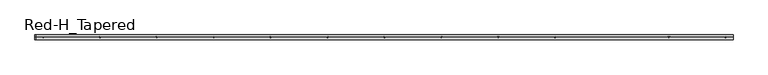
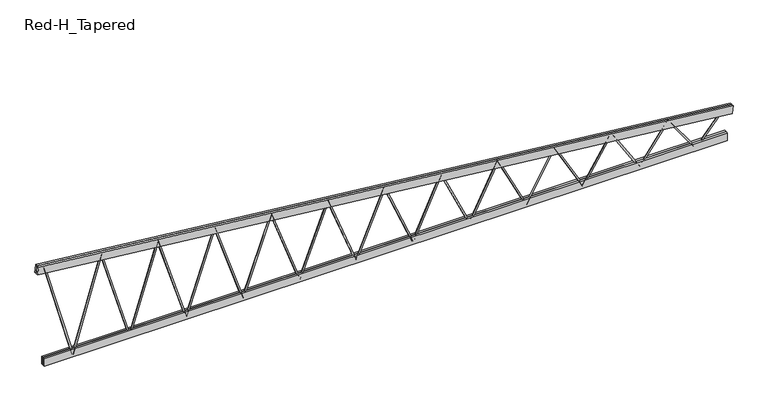
"""IFC4 building model written with IfcOpenShell, lengths in millimetres: beam geometry, Construction_Frames_RedBuilt_Openweb_Red-H_Tapered : Red-H_Tapered."""

from ifc_helpers import new_model, si_unit, point, frame, origin, origin_2d, place, context, project, spatial, polyline, circle_curve, trimmed, segment, composite_curve, outline, extrude, source, transform, mapped, element, save


def red_h_tapered_72d70656(model_context):
    return source(origin(), model_context, "Body", "SweptSolid", [
        extrude(outline(composite_curve([segment(trimmed(circle_curve(origin_2d(), 12.7), [point((0.0, -12.7000001))], [point((0.0, 12.7))], False, "CARTESIAN"), True, "CONTINUOUS"), segment(trimmed(circle_curve(origin_2d(), 12.7), [point((0.0, 12.7))], [point((0.0, -12.7000001))], False, "CARTESIAN"), True, "CONTINUOUS")], self_intersect=False)), frame((-495.696875, 0.0, -367.0101562), z_axis=(-0.36126696231281513, 0.0, 0.9324624292384498), x_axis=(0.0, -1.0, 0.0)), (0.0, 0.0, 1.0), 1372.1068537),
        extrude(outline(composite_curve([segment(trimmed(circle_curve(origin_2d(), 12.7), [point((0.0, 12.7000001))], [point((0.0, -12.7))], False, "CARTESIAN"), True, "CONTINUOUS"), segment(trimmed(circle_curve(origin_2d(), 12.7), [point((0.0, -12.7))], [point((0.0, 12.7000001))], False, "CARTESIAN"), True, "CONTINUOUS")], self_intersect=False)), frame((-1487.090625, 0.0, -367.0101562), z_axis=(0.3612669623128153, 0.0, 0.9324624292384498), x_axis=(0.0, -1.0, 0.0)), (0.0, 0.0, 1.0), 1372.1068537),
        extrude(outline(composite_curve([segment(trimmed(circle_curve(origin_2d(), 12.7), [point((0.0, -12.7000001))], [point((0.0, 12.7))], False, "CARTESIAN"), True, "CONTINUOUS"), segment(trimmed(circle_curve(origin_2d(), 12.7), [point((0.0, 12.7))], [point((0.0, -12.7000001))], False, "CARTESIAN"), True, "CONTINUOUS")], self_intersect=False)), frame((-1487.090625, 0.0, -367.0101562), z_axis=(-0.33832311058632253, 0.0, 0.9410300063458099), x_axis=(0.0, -1.0, 0.0)), (0.0, 0.0, 1.0), 1465.158186),
        extrude(outline(composite_curve([segment(trimmed(circle_curve(origin_2d(), 12.7), [point((0.0, -12.7))], [point((0.0, 12.7000001))], False, "CARTESIAN"), True, "CONTINUOUS"), segment(trimmed(circle_curve(origin_2d(), 12.7), [point((0.0, 12.7000001))], [point((0.0, -12.7))], False, "CARTESIAN"), True, "CONTINUOUS")], self_intersect=False)), frame((-2478.484375, 0.0, -367.0101562), z_axis=(0.3383231105863266, 0.0, 0.9410300063458085), x_axis=(0.0, -1.0, 0.0)), (0.0, 0.0, 1.0), 1465.158186),
        extrude(outline(composite_curve([segment(trimmed(circle_curve(origin_2d(), 12.7), [point((0.0, 12.7))], [point((0.0, -12.7))], False, "CARTESIAN"), True, "CONTINUOUS"), segment(trimmed(circle_curve(origin_2d(), 12.7), [point((0.0, -12.7))], [point((0.0, 12.7))], False, "CARTESIAN"), True, "CONTINUOUS")], self_intersect=False)), frame((-2478.484375, 0.0, -367.0101562), z_axis=(-0.3179616527746543, 0.0, 0.9481035741757387), x_axis=(0.0, -1.0, 0.0)), (0.0, 0.0, 1.0), 1558.9832003),
        extrude(outline(composite_curve([segment(trimmed(circle_curve(origin_2d(), 12.7), [point((0.0, -12.7))], [point((0.0, 12.7))], False, "CARTESIAN"), True, "CONTINUOUS"), segment(trimmed(circle_curve(origin_2d(), 12.7), [point((0.0, 12.7))], [point((0.0, -12.7))], False, "CARTESIAN"), True, "CONTINUOUS")], self_intersect=False)), frame((-3469.878125, 0.0, -367.0101562), z_axis=(0.3179616527746538, 0.0, 0.9481035741757388), x_axis=(0.0, -1.0, 0.0)), (0.0, 0.0, 1.0), 1558.9832003),
        extrude(outline(composite_curve([segment(trimmed(circle_curve(origin_2d(), 12.7), [point((0.0, 12.6999999))], [point((0.0, -12.7))], False, "CARTESIAN"), True, "CONTINUOUS"), segment(trimmed(circle_curve(origin_2d(), 12.7), [point((0.0, -12.7))], [point((0.0, 12.6999999))], False, "CARTESIAN"), True, "CONTINUOUS")], self_intersect=False)), frame((-3469.878125, 0.0, -367.0101562), z_axis=(-0.29979546818875297, 0.0, 0.9540034996023267), x_axis=(0.0, -1.0, 0.0)), (0.0, 0.0, 1.0), 1653.4501939),
        extrude(outline(composite_curve([segment(trimmed(circle_curve(origin_2d(), 12.7), [point((0.0, -12.6999999))], [point((0.0, 12.7))], False, "CARTESIAN"), True, "CONTINUOUS"), segment(trimmed(circle_curve(origin_2d(), 12.7), [point((0.0, 12.7))], [point((0.0, -12.6999999))], False, "CARTESIAN"), True, "CONTINUOUS")], self_intersect=False)), frame((-4461.271875, 0.0, -367.0101562), z_axis=(0.29979546818875863, 0.0, 0.9540034996023249), x_axis=(0.0, -1.0, 0.0)), (0.0, 0.0, 1.0), 1653.4501939),
        extrude(outline(composite_curve([segment(trimmed(circle_curve(origin_2d(), 12.7), [point((0.0, 12.6999999))], [point((0.0, -12.7))], False, "CARTESIAN"), True, "CONTINUOUS"), segment(trimmed(circle_curve(origin_2d(), 12.7), [point((0.0, -12.7))], [point((0.0, 12.6999999))], False, "CARTESIAN"), True, "CONTINUOUS")], self_intersect=False)), frame((-4461.271875, 0.0, -367.0101562), z_axis=(-0.28350563367982917, 0.0, 0.9589705708059025), x_axis=(0.0, -1.0, 0.0)), (0.0, 0.0, 1.0), 1748.4551138),
        extrude(outline(composite_curve([segment(trimmed(circle_curve(origin_2d(), 12.7), [point((0.0, -12.6999999))], [point((0.0, 12.7))], False, "CARTESIAN"), True, "CONTINUOUS"), segment(trimmed(circle_curve(origin_2d(), 12.7), [point((0.0, 12.7))], [point((0.0, -12.6999999))], False, "CARTESIAN"), True, "CONTINUOUS")], self_intersect=False)), frame((-5452.665625, 0.0, -367.0101562), z_axis=(0.28350563367982784, 0.0, 0.958970570805903), x_axis=(0.0, -1.0, 0.0)), (0.0, 0.0, 1.0), 1748.4551138),
        extrude(outline(composite_curve([segment(trimmed(circle_curve(origin_2d(), 12.7), [point((0.0, 12.7))], [point((0.0, -12.7))], False, "CARTESIAN"), True, "CONTINUOUS"), segment(trimmed(circle_curve(origin_2d(), 12.7), [point((0.0, -12.7))], [point((0.0, 12.7))], False, "CARTESIAN"), True, "CONTINUOUS")], self_intersect=False)), frame((-5452.665625, 0.0, -367.0101562), z_axis=(-0.2688285115613956, 0.0, 0.9631880560781911), x_axis=(0.0, -1.0, 0.0)), (0.0, 0.0, 1.0), 1843.9148144),
        extrude(outline(composite_curve([segment(trimmed(circle_curve(origin_2d(), 12.7), [point((0.0, 12.7))], [point((0.0, -12.7))], False, "CARTESIAN"), True, "CONTINUOUS"), segment(trimmed(circle_curve(origin_2d(), 12.7), [point((0.0, -12.7))], [point((0.0, 12.7))], False, "CARTESIAN"), True, "CONTINUOUS")], self_intersect=False)), frame((5452.665625, 0.0, -367.0101562), z_axis=(0.6469865747482126, 0.0, 0.7625013915368125), x_axis=(0.0, -1.0, 0.0)), (0.0, 0.0, 1.0), 766.1625362),
        extrude(outline(composite_curve([segment(trimmed(circle_curve(origin_2d(), 12.7), [point((0.0, -12.7))], [point((0.0, 12.7))], False, "CARTESIAN"), True, "CONTINUOUS"), segment(trimmed(circle_curve(origin_2d(), 12.7), [point((0.0, 12.7))], [point((0.0, -12.7))], False, "CARTESIAN"), True, "CONTINUOUS")], self_intersect=False)), frame((5452.665625, 0.0, -367.0101562), z_axis=(-0.5870801868170475, 0.0, 0.8095287853108502), x_axis=(0.0, -1.0, 0.0)), (0.0, 0.0, 1.0), 844.3427084),
        extrude(outline(composite_curve([segment(trimmed(circle_curve(origin_2d(), 12.7), [point((0.0, 12.7))], [point((0.0, -12.7))], False, "CARTESIAN"), True, "CONTINUOUS"), segment(trimmed(circle_curve(origin_2d(), 12.7), [point((0.0, -12.7))], [point((0.0, 12.7))], False, "CARTESIAN"), True, "CONTINUOUS")], self_intersect=False)), frame((4461.271875, 0.0, -367.0101562), z_axis=(0.5870801868170453, 0.0, 0.8095287853108518), x_axis=(0.0, -1.0, 0.0)), (0.0, 0.0, 1.0), 844.3427084),
        extrude(outline(composite_curve([segment(trimmed(circle_curve(origin_2d(), 12.7), [point((0.0, -12.7))], [point((0.0, 12.7))], False, "CARTESIAN"), True, "CONTINUOUS"), segment(trimmed(circle_curve(origin_2d(), 12.7), [point((0.0, 12.7))], [point((0.0, -12.7))], False, "CARTESIAN"), True, "CONTINUOUS")], self_intersect=False)), frame((4461.271875, 0.0, -367.0101562), z_axis=(-0.534973937894613, 0.0, 0.8448685612410554), x_axis=(0.0, -1.0, 0.0)), (0.0, 0.0, 1.0), 926.5813526),
        extrude(outline(composite_curve([segment(trimmed(circle_curve(origin_2d(), 12.7), [point((0.0, 12.7))], [point((0.0, -12.7))], False, "CARTESIAN"), True, "CONTINUOUS"), segment(trimmed(circle_curve(origin_2d(), 12.7), [point((0.0, -12.7))], [point((0.0, 12.7))], False, "CARTESIAN"), True, "CONTINUOUS")], self_intersect=False)), frame((3469.878125, 0.0, -367.0101562), z_axis=(0.5349739378946109, 0.0, 0.8448685612410566), x_axis=(0.0, -1.0, 0.0)), (0.0, 0.0, 1.0), 926.5813526),
        extrude(outline(composite_curve([segment(trimmed(circle_curve(origin_2d(), 12.7), [point((0.0, -12.7))], [point((0.0, 12.7))], False, "CARTESIAN"), True, "CONTINUOUS"), segment(trimmed(circle_curve(origin_2d(), 12.7), [point((0.0, 12.7))], [point((0.0, -12.7))], False, "CARTESIAN"), True, "CONTINUOUS")], self_intersect=False)), frame((3469.878125, 0.0, -367.0101562), z_axis=(-0.4898725706476443, 0.0, 0.8717940493758081), x_axis=(0.0, -1.0, 0.0)), (0.0, 0.0, 1.0), 1011.8894274),
        extrude(outline(composite_curve([segment(trimmed(circle_curve(origin_2d(), 12.7), [point((0.0, 12.7))], [point((0.0, -12.7))], False, "CARTESIAN"), True, "CONTINUOUS"), segment(trimmed(circle_curve(origin_2d(), 12.7), [point((0.0, -12.7))], [point((0.0, 12.7))], False, "CARTESIAN"), True, "CONTINUOUS")], self_intersect=False)), frame((2478.484375, 0.0, -367.0101562), z_axis=(0.48987257064764494, 0.0, 0.8717940493758077), x_axis=(0.0, -1.0, 0.0)), (0.0, 0.0, 1.0), 1011.8894274),
        extrude(outline(composite_curve([segment(trimmed(circle_curve(origin_2d(), 12.7), [point((0.0, -12.7))], [point((0.0, 12.7))], False, "CARTESIAN"), True, "CONTINUOUS"), segment(trimmed(circle_curve(origin_2d(), 12.7), [point((0.0, 12.7))], [point((0.0, -12.7))], False, "CARTESIAN"), True, "CONTINUOUS")], self_intersect=False)), frame((2478.484375, 0.0, -367.0101562), z_axis=(-0.4508168226533229, 0.0, 0.8926164867471149), x_axis=(0.0, -1.0, 0.0)), (0.0, 0.0, 1.0), 1099.5527454),
        extrude(outline(composite_curve([segment(trimmed(circle_curve(origin_2d(), 12.7), [point((0.0, 12.7))], [point((0.0, -12.7))], False, "CARTESIAN"), True, "CONTINUOUS"), segment(trimmed(circle_curve(origin_2d(), 12.7), [point((0.0, -12.7))], [point((0.0, 12.7))], False, "CARTESIAN"), True, "CONTINUOUS")], self_intersect=False)), frame((1487.090625, 0.0, -367.0101562), z_axis=(0.450816822653327, 0.0, 0.8926164867471128), x_axis=(0.0, -1.0, 0.0)), (0.0, 0.0, 1.0), 1099.5527454),
        extrude(outline(composite_curve([segment(trimmed(circle_curve(origin_2d(), 12.7), [point((0.0, -12.7))], [point((0.0, 12.7))], False, "CARTESIAN"), True, "CONTINUOUS"), segment(trimmed(circle_curve(origin_2d(), 12.7), [point((0.0, 12.7))], [point((0.0, -12.7))], False, "CARTESIAN"), True, "CONTINUOUS")], self_intersect=False)), frame((1487.090625, 0.0, -367.0101562), z_axis=(-0.4168846289839184, 0.0, 0.9089594083989344), x_axis=(0.0, -1.0, 0.0)), (0.0, 0.0, 1.0), 1189.0504963),
        extrude(outline(composite_curve([segment(trimmed(circle_curve(origin_2d(), 12.7), [point((0.0, 12.7))], [point((0.0, -12.7))], False, "CARTESIAN"), True, "CONTINUOUS"), segment(trimmed(circle_curve(origin_2d(), 12.7), [point((0.0, -12.7))], [point((0.0, 12.7))], False, "CARTESIAN"), True, "CONTINUOUS")], self_intersect=False)), frame((495.696875, 0.0, -367.0101562), z_axis=(0.41688462898391915, 0.0, 0.9089594083989341), x_axis=(0.0, -1.0, 0.0)), (0.0, 0.0, 1.0), 1189.0504963),
        extrude(outline(composite_curve([segment(trimmed(circle_curve(origin_2d(), 12.7), [point((0.0, -12.7000001))], [point((0.0, 12.7))], False, "CARTESIAN"), True, "CONTINUOUS"), segment(trimmed(circle_curve(origin_2d(), 12.7), [point((0.0, 12.7))], [point((0.0, -12.7000001))], False, "CARTESIAN"), True, "CONTINUOUS")], self_intersect=False)), frame((495.696875, 0.0, -367.0101562), z_axis=(-0.38726380498396673, 0.0, 0.9219689503173847), x_axis=(0.0, -1.0, 0.0)), (0.0, 0.0, 1.0), 1279.9979462),
        extrude(outline(composite_curve([segment(trimmed(circle_curve(origin_2d(), 12.7), [point((0.0, 12.7000001))], [point((0.0, -12.7))], False, "CARTESIAN"), True, "CONTINUOUS"), segment(trimmed(circle_curve(origin_2d(), 12.7), [point((0.0, -12.7))], [point((0.0, 12.7000001))], False, "CARTESIAN"), True, "CONTINUOUS")], self_intersect=False)), frame((-495.696875, 0.0, -367.0101562), z_axis=(0.38726380498393514, 0.0, 0.921968950317398), x_axis=(0.0, -1.0, 0.0)), (0.0, 0.0, 1.0), 1279.9979462),
        extrude(outline(polyline([(-5973.7625, -41.275), (-5973.7625, -3.175), (5973.7625, -3.175), (5973.7625, -41.275), (-5973.7625, -41.275)])), frame((0.0, 0.0, -386.0601562), z_axis=(0.0, 0.0, 1.0), x_axis=(1.0, 0.0, 0.0)), (0.0, 0.0, 1.0), 139.7),
        extrude(outline(polyline([(-5973.7625, 3.175), (-5973.7625, 41.275), (5973.7625, 41.275), (5973.7625, 3.175), (-5973.7625, 3.175)])), frame((0.0, 0.0, -386.0601562), z_axis=(0.0, 0.0, 1.0), x_axis=(1.0, 0.0, 0.0)), (0.0, 0.0, 1.0), 139.7),
        extrude(outline(polyline([(0.0, -38.1), (0.0, 0.0), (12216.092656, 0.0), (12216.092656, -38.1), (0.0, -38.1)])), frame((-6089.7951125, -3.175, 1346.649871), z_axis=(0.10331147082303982, 0.0, 0.9946490536849569), x_axis=(0.9946490536849569, 0.0, -0.10331147082303982)), (0.0, 0.0, 1.0), 139.7),
        extrude(outline(polyline([(0.0, -38.1), (0.0, 0.0), (12216.092656, 0.0), (12216.092656, -38.1), (0.0, -38.1)])), frame((-6089.7951125, 41.275, 1346.649871), z_axis=(0.10331147082303982, 0.0, 0.9946490536849569), x_axis=(0.9946490536849569, 0.0, -0.10331147082303982)), (0.0, 0.0, 1.0), 139.7),
    ])


if __name__ == "__main__":
    model = new_model("IFC4")
    model_context = context("Model", 3, world=origin())
    ifc_project = project(units=[si_unit("LENGTHUNIT", "METRE", prefix="MILLI")], contexts=[model_context])
    site = spatial("IfcSite", under=ifc_project)
    building = spatial("IfcBuilding", under=site)
    placement = place(None, origin())
    red_h_tapered_shape = red_h_tapered_72d70656(model_context)
    element("IfcBeam", 1, ObjectType="Construction_Frames_RedBuilt_Openweb_Red-H_Tapered : Red-H_Tapered", at=placement, inside=building, context=model_context, shape_type="MappedRepresentation", body=[
        mapped(red_h_tapered_shape, transform((0.0, 0.0, 0.0), x_axis=(1.0, 0.0, 0.0), y_axis=(0.0, 1.0, 0.0), z_axis=(0.0, 0.0, 1.0))),
    ])
    save(model, "model.ifc")

# Revit data of these elements
# Type "Construction_Frames_RedBuilt_Openweb_Red-H_Tapered : Red-H_Tapered"
#   Youtube clip = ""
#   Weight Net (Kg) = "0"
#   Webs = "Up to 2\" diameter tubular steel"
#   Uniformat II Description = ""
#   Uniformat II Code = ""
#   Uniclass 2015 Name = "Softwood trusses"
#   Uniclass 2015 Code = "Pr_20_85_90_81"
#   Uniclass 2.0 Description = "Structural Framing Systems"
#   Uniclass 2.0 Code = "SS-15-10-75"
#   Uniclass 1.4 Description = "Trusses"
#   Uniclass 1.4 Code = "L3523"
#   UNSPSC Code = "30103606"
#   Technical description = "http://www.redbuilt.com/reference/literature-and-other-resources"
#   Region South America = "None"
#   Region Oceania = "None"
#   Region North America = "US"
#   Region Middle East = "None"
#   Region Europe = "None"
#   Region Asia = "None"
#   Region Antarctica = "None"
#   Region Africa = "None"
#   QR code = "http://bimobject.com/redbuilt/product/redbuilt-0003"
#   Product url = "http://www.redbuilt.com/products/default.aspx?id=2"
#   Product group = "Wood Trusses"
#   Product family = "Construction"
#   Product data url = "https://bimobject.com/redbuilt/product/redbuilt-0003"
#   Product certification = ""
#   Product SKU = "redbuilt-0003"
#   Product Page URL = "http://www.redbuilt.com/commercial-systems/red-m-red-h-open-web-trusses"
#   Product Guid = "2c5793f2-6ffb-4665-b825-cf90c048e711"
#   Product Documentation Link = "http://www.redbuilt.com/documents/OW_Guide_2017_07_LowRes_wLinks.pdf"
#   OmniClass Description = "Wood Trusses"
#   OmniClass Code = "23-13 35 19 13 17"
#   NBS Reference Description = ""
#   NBS Reference Code = ""
#   Material secondary = "Steel"
#   Material main = "Wood"
#   Masterformat 2014 Description = "Metal-Web Wood Joists"
#   Masterformat 2014 Code = "06 17 36"
#   Manufacturer name = "RedBuilt"
#   Manufacturer country = "United States"
#   Installation instructions = "http://www.redbuilt.com/documents/Installation_Sheets_Open-Web.pdf"
#   IFC Classification = ""
#   EAN code = ""
#   Design country = "United States"
#   Product Information = "http://redbuilt.com/products/default.aspx?id=2"
#   Model = "Red-H-Tapered"
#   Manufacturer URL = "http://redbuilt.com/"
#   Manufacturer = "RedBuilt™"
#   Description = "Open Web Truss"
#   Date of publishing = "8/17/2010"
#   Contact us = "http://redbuilt.com/contact/"
#   Chords = "Double 1½\" x 5½\" MSR lumber"
#   COBIe Type Category = ""
#   Brand url = "http://www.redbuilt.com"
#   BIMobject main category code = "construction"
#   BIMobject main category = "Construction"
#   BIMobject category code = "construction-frames-trusses"
#   BIMobject category = "Frames & Trusses"
#   Web Radius = 0' - 0 1/2"
#   Web Layout Offset Start [instance default] = 0' - 5"
#   Web Layout Offset End [instance default] = 0' - 5"
#   Web Diameter = 0' - 1"
#   TotalLength [instance default] = 20' - 0"
#   Span Minimum = 4' - 0"
#   Span Maximum = 70' - 0"
#   Span Limit [instance default] = 20' - 0"
#   Nominal width = 0' - 0"
#   Nominal height = 0' - 0"
#   Inner Depth Top [instance default] = 0' - 2.76372"
#   Depth Start [instance default] = 6' - 0"
#   Top Chord Length [instance default] = 20' - 1.19701"
#   TC Extension Start Aux [instance default] = 0' - 0"
#   TC Extension End Aux [instance default] = 0' - 0"
#   T-B Chord Length Difference L [instance default] = 0' - 4"
#   T-B Chord Length Difference [instance default] = 0' - 4"
#   Height 2 [instance default] = 6' - 0"
#   Depth Minimum at Wall = 2' - 0"
#   Depth Maximum at Wall = 6' - 0"
#   Depth Lower End [instance default] = 2' - 0"
#   Depth Higher End [instance default] = 6' - 0"
#   Depth End [instance default] = 2' - 0"
#   Depth 2 [instance default] = 2' - 0"
#   Chord Width = 0' - 3 1/4"
#   Chord Thickness = 0' - 1 1/2"
#   Chord Depth = 0' - 5 1/2"
#   Offset Start [instance default] = 0' - 0"
#   TC Extension Start [instance default] = 0' - 0"
#   End Panel = 0' - 5"
#   Offset End [instance default] = 0' - 0"
#   TC Extension End [instance default] = 0' - 0"
#   Length [instance default] = 20' - 0"
#   Angle [instance default] = 5.71059°
#   Span Limit Warning [instance default] = no
#   Edition number = 1
#   Top Bearing Start [instance default] = yes
#   Top Bearing End [instance default] = yes
#   Bottom Bearing Start [instance default] = no
#   Bottom Bearing End [instance default] = no
#   8 Panels [instance default] = yes
#   16 Panels [instance default] = no
#   12 Panels [instance default] = no
#   Web Material = RedBuilt-Steel, Galvanized
#   Clip Material = RedBuilt-Steel, Galvanized
#   Chords Material = RedBuilt-MSR
#   URL = ""
#   Assembly Code = ""
# Element 1 (IfcBeam, "Construction_Frames_RedBuilt_Openweb_Red-H_Tapered : Red-H_Tapered")
#   TotalLength = 39' - 10 3/8"
#   Span Limit = 39' - 10 3/8"
#   Inner Depth Top = 0' - 2.76479"
#   Top Chord Length = 40' - 0.94853"
#   Depth 2 = 4' - 1 11/16"
#   Angle = 5.92989°
#   8 Panels = no
#   12 Panels = yes
#   Materials on its faces: "RedBuilt-Steel, Galvanized", "RedBuilt-MSR"
# Materials
#   "RedBuilt-Steel, Galvanized": class "Metal", colour RGB 164 172 176, transparency 0, Manufacturer = "RedBuilt. LLC", Comments = "Openweb Metal Web", URL = "http://www.redbuilt.com/", Description = "Galvanized steel", Cost = 0
#   "RedBuilt-MSR": class "Wood", colour RGB 213 182 136, transparency 0, Manufacturer = "RedBuilt, LLC", URL = "http://www.redbuilt.com/", Cost = 0
